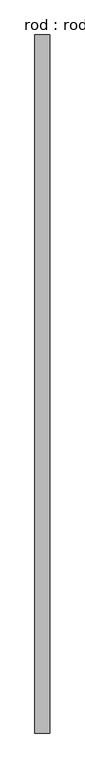
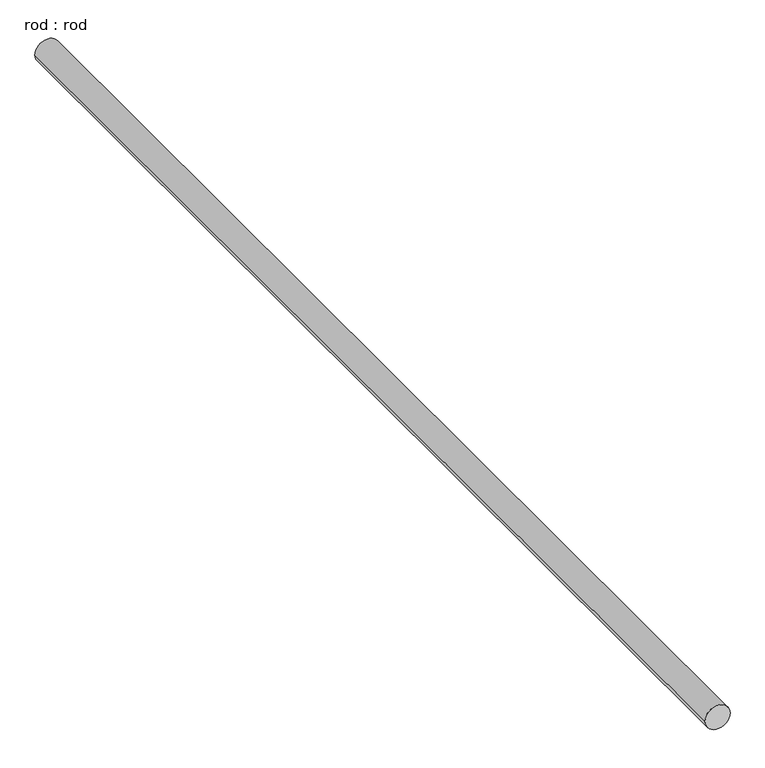
"""IFC4 building model written with IfcOpenShell, lengths in millimetres: proxy geometry, rod : rod."""

from ifc_helpers import new_model, si_unit, point, frame, frame_2d, origin, place, context, project, spatial, circle_curve, trimmed, segment, composite_curve, outline, extrude, source, transform, mapped, element, save


def rod_rod_bbb09cc0(model_context):
    return source(origin(), model_context, "Body", "SweptSolid", [
        extrude(outline(composite_curve([segment(trimmed(circle_curve(frame_2d((0.0108462, 0.0)), 200.0), [point((0.0108462, 200.0))], [point((0.0108462, -200.0))], False, "CARTESIAN"), True, "CONTINUOUS"), segment(trimmed(circle_curve(frame_2d((0.0108462, 0.0)), 200.0), [point((0.0108462, -200.0))], [point((0.0108462, 200.0))], False, "CARTESIAN"), True, "CONTINUOUS")], self_intersect=False)), frame((0.0, -5185.0491624, 0.0), z_axis=(0.0, 1.0, 0.0), x_axis=(0.0, 0.0, 1.0)), (0.0, 0.0, 1.0), 18555.5555556),
    ])


if __name__ == "__main__":
    model = new_model("IFC4")
    model_context = context("Model", 3, world=origin())
    ifc_project = project(units=[si_unit("LENGTHUNIT", "METRE", prefix="MILLI")], contexts=[model_context])
    site = spatial("IfcSite", under=ifc_project)
    building = spatial("IfcBuilding", under=site)
    placement = place(None, origin())
    rod_rod_shape = rod_rod_bbb09cc0(model_context)
    element("IfcBuildingElementProxy", 1, Name="rod : rod", ObjectType="rod : rod", at=placement, inside=building, context=model_context, shape_type="MappedRepresentation", body=[
        mapped(rod_rod_shape, transform((0.0, 0.0, 0.0), x_axis=(1.0, 0.0, 0.0), y_axis=(0.0, 1.0, 0.0), z_axis=(0.0, 0.0, 1.0))),
    ])
    save(model, "model.ifc")

# Revit data of these elements
# Type "rod : rod"
#   Default Elevation = 0
